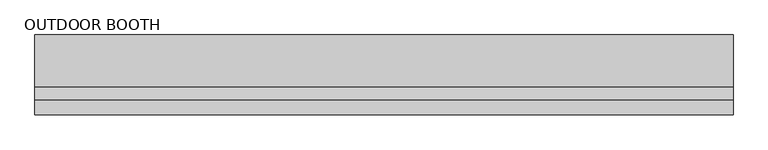
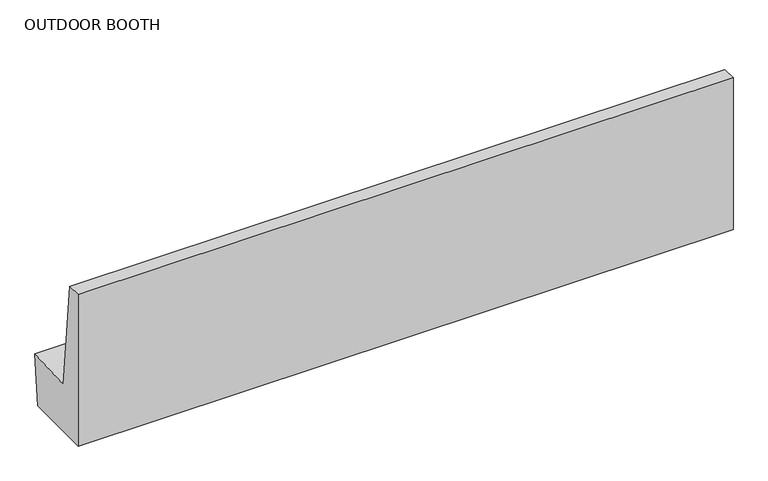
"""IFC4 building model written with IfcOpenShell, lengths in millimetres: furniture geometry, OD_CW_Booth : OUTDOOR BOOTH."""

from ifc_helpers import new_model, si_unit, frame, origin, place, context, project, spatial, polyline, outline, extrude, source, transform, mapped, element, save


def outdoor_booth_872b75e5(model_context):
    return source(origin(), model_context, "Body", "SweptSolid", [
        extrude(outline(polyline([(-609.6, 1397.0), (-484.4524721, 1397.0), (-382.9385128, 431.1591941), (43.0849153, 453.4861359), (3.4100193, 0.0), (-609.6, 0.0), (-609.6, 1397.0)])), frame((18.7377049, 0.0, 0.0), z_axis=(1.0, 0.0, 0.0), x_axis=(0.0, 1.0, 0.0)), (0.0, 0.0, 1.0), 5700.9355441),
    ])


if __name__ == "__main__":
    model = new_model("IFC4")
    model_context = context("Model", 3, world=origin())
    ifc_project = project(units=[si_unit("LENGTHUNIT", "METRE", prefix="MILLI")], contexts=[model_context])
    site = spatial("IfcSite", under=ifc_project)
    building = spatial("IfcBuilding", under=site)
    placement = place(None, origin())
    outdoor_booth_shape = outdoor_booth_872b75e5(model_context)
    element("IfcFurniture", 1, ObjectType="OD_CW_Booth : OUTDOOR BOOTH", at=placement, inside=building, context=model_context, shape_type="MappedRepresentation", body=[
        mapped(outdoor_booth_shape, transform((0.0, 0.0, 0.0), x_axis=(1.0, 0.0, 0.0), y_axis=(0.0, 1.0, 0.0), z_axis=(0.0, 0.0, 1.0))),
    ])
    save(model, "model.ifc")

# Revit data of these elements
# Type "OD_CW_Booth : OUTDOOR BOOTH"
#   Type Mark = "TYPE-OUTDOOR"
#   Width = 4' - 0"
#   OD_CW_Width [instance default] = 2' - 10"
#   OD_CW_Length [instance default] = 26' - 1 83/256"
#   OD_CW_Height [instance default] = 2' - 3"
#   Height = 3' - 0"
#   Depth = 2' - 0"
#   Seating Count [instance default] = 10
#   OD_CW_Material_Front Panel [instance default] = none
#   OD_CW_Material_Body [instance default] = none
# Element 1 (IfcFurniture, "OD_CW_Booth : OUTDOOR BOOTH")
#   OD_CW_Length = 18' - 8.44628"
#   Seating Count = 7
#   OD_CW_Material_Body = Sals Wood
#   Materials on its faces: "Sals Wood"
# Materials
#   "Sals Wood": class "Wood", colour RGB 198 202 183, transparency 0, Description = "Generic wood", Cost = 0
